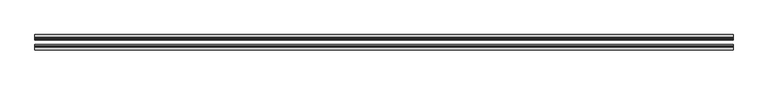
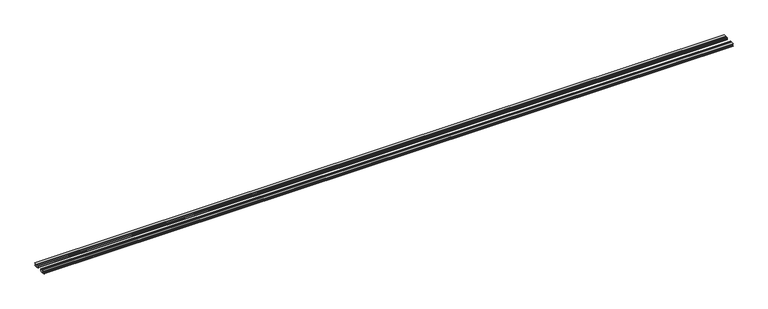
"""IFC4 building model written with IfcOpenShell, lengths in millimetres: proxy geometry, Generic Models 6:Generic Models 2:318829:Generic Models 2:318829 : Generic Models 6:Generic Models 2:318829:6 : Generic Models 6:Generic Models 2:318829:Generic Models 2:318829 : Generic Models 6:Generic Models 2:318829:300683."""

from ifc_helpers import new_model, si_unit, frame, origin, place, context, project, spatial, polyline, outline, extrude, source, transform, mapped, element, save


def generic_models_35608d38(model_context):
    return source(origin(), model_context, "Body", "SweptSolid", [
        extrude(outline(polyline([(-536510.30862, 10113.491026), (-536519.1107582, 10113.491026), (-536518.5446453, 10114.9396708), (-536518.0741162, 10118.253526), (-536518.5446453, 10121.5673812), (-536519.1107582, 10123.016026), (-536510.30862, 10123.016026), (-536512.6984451, 10121.6918427), (-536514.1597526, 10119.8297666), (-536514.4639345, 10117.7211022), (-536513.5634042, 10115.6957305), (-536511.5990415, 10114.0705024), (-536510.30862, 10113.491026)])), frame((591391.6367242, 0.0, 0.0), z_axis=(1.0, 0.0, 0.0), x_axis=(0.0, 1.0, 0.0)), (0.0, 0.0, 1.0), 2438.4),
        extrude(outline(polyline([(-536505.1735447, 10113.6104318), (-536506.7631787, 10113.491026), (-536508.3528126, 10113.6104318), (-536511.2172339, 10114.5300536), (-536513.199475, 10116.1871547), (-536513.9069287, 10118.253526), (-536513.199475, 10120.3198973), (-536511.2172339, 10121.9769984), (-536508.3528126, 10122.8966202), (-536506.7631787, 10123.016026), (-536505.1735447, 10122.8966202), (-536502.3091234, 10121.9769984), (-536500.3268823, 10120.3198973), (-536499.6194287, 10118.253526), (-536500.3268823, 10116.1871547), (-536502.3091234, 10114.5300536), (-536505.1735447, 10113.6104318)])), frame((591391.6367242, 0.0, 0.0), z_axis=(1.0, 0.0, 0.0), x_axis=(0.0, 1.0, 0.0)), (0.0, 0.0, 1.0), 2438.4),
        extrude(outline(polyline([(-536474.0353623, 10113.491026), (-536472.7449409, 10114.0705024), (-536470.7805781, 10115.6957305), (-536469.8800479, 10117.7211022), (-536470.1842297, 10119.8297666), (-536471.6455372, 10121.6918427), (-536474.0353623, 10123.016026), (-536465.2332241, 10123.016026), (-536465.7993371, 10121.5673812), (-536466.2698662, 10118.253526), (-536465.7993371, 10114.9396708), (-536465.2332241, 10113.491026), (-536474.0353623, 10113.491026)])), frame((591391.6367242, 0.0, 0.0), z_axis=(1.0, 0.0, 0.0), x_axis=(0.0, 1.0, 0.0)), (0.0, 0.0, 1.0), 2438.4),
        extrude(outline(polyline([(-536479.1704376, 10113.6104318), (-536482.034859, 10114.5300536), (-536484.0171, 10116.1871547), (-536484.7245537, 10118.253526), (-536484.0171, 10120.3198973), (-536482.034859, 10121.9769984), (-536479.1704376, 10122.8966202), (-536477.5808037, 10123.016026), (-536475.9911698, 10122.8966202), (-536473.1267484, 10121.9769984), (-536471.1445073, 10120.3198973), (-536470.4370537, 10118.253526), (-536471.1445073, 10116.1871547), (-536473.1267484, 10114.5300536), (-536475.9911698, 10113.6104318), (-536477.5808037, 10113.491026), (-536479.1704376, 10113.6104318)])), frame((591391.6367242, 0.0, 0.0), z_axis=(1.0, 0.0, 0.0), x_axis=(0.0, 1.0, 0.0)), (0.0, 0.0, 1.0), 2438.4),
    ])


if __name__ == "__main__":
    model = new_model("IFC4")
    model_context = context("Model", 3, world=origin())
    ifc_project = project(units=[si_unit("LENGTHUNIT", "METRE", prefix="MILLI")], contexts=[model_context])
    site = spatial("IfcSite", under=ifc_project)
    building = spatial("IfcBuilding", under=site)
    placement = place(None, origin())
    generic_models_shape = generic_models_35608d38(model_context)
    element("IfcBuildingElementProxy", 1, Name="Generic Models 6:Generic Models 2:318829:Generic Models 2:318829 : Generic Models 6:Generic Models 2:318829:6 : Generic Models 6:Generic Models 2:318829:Generic Models 2:318829 : Generic Models 6:Generic Models 2:318829:300683", ObjectType="Generic Models 6:Generic Models 2:318829:Generic Models 2:318829 : Generic Models 6:Generic Models 2:318829:6 : Generic Models 6:Generic Models 2:318829:Generic Models 2:318829 : Generic Models 6:Generic Models 2:318829:300683", at=placement, inside=building, context=model_context, shape_type="MappedRepresentation", body=[
        mapped(generic_models_shape, transform((0.0, 0.0, 0.0), x_axis=(1.0, 0.0, 0.0), y_axis=(0.0, 1.0, 0.0), z_axis=(0.0, 0.0, 1.0))),
    ])
    save(model, "model.ifc")

# Revit data of these elements
# Type "Generic Models 6:Generic Models 2:318829:Generic Models 2:318829 : Generic Models 6:Generic Models 2:318829:6 : Generic Models 6:Generic Models 2:318829:Generic Models 2:318829 : Generic Models 6:Generic Models 2:318829:300683"
#   NameOverride = "Generic Models 6:Generic Models 2:318829:Generic Models 2:318829 : Generic Models 6:Generic Models 2:318829:300683"
#   ObjectTypeOverride = "Generic Models 2:318829 : Generic Models 6:Generic Models 2:318829"
#   Reference = "Generic Models 2"
#   Tag = "300683"
# Element 1 (IfcBuildingElementProxy, "Generic Models 6:Generic Models 2:318829:Generic Models 2:318829 : Generic Models 6:Generic Models 2:318829:6 : Generic Models 6:Generic Models 2:318829:Generic Models 2:318829 : Generic Models 6:Generic Models 2:318829:300683")
#   Materials on its faces: "SEALANT & BACKER ROD"
# Materials
#   "SEALANT & BACKER ROD": class "Unassigned", colour RGB 120 120 120, transparency 0, Cost = 0
